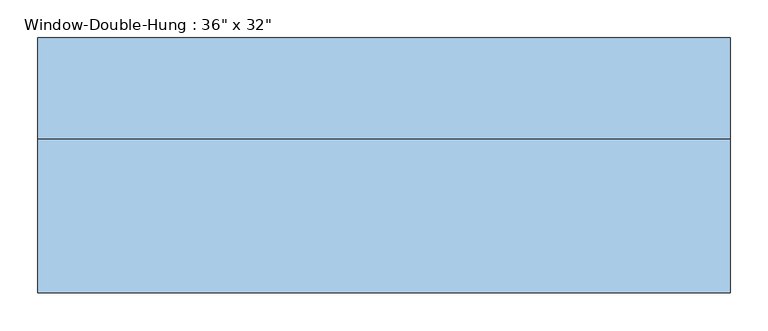
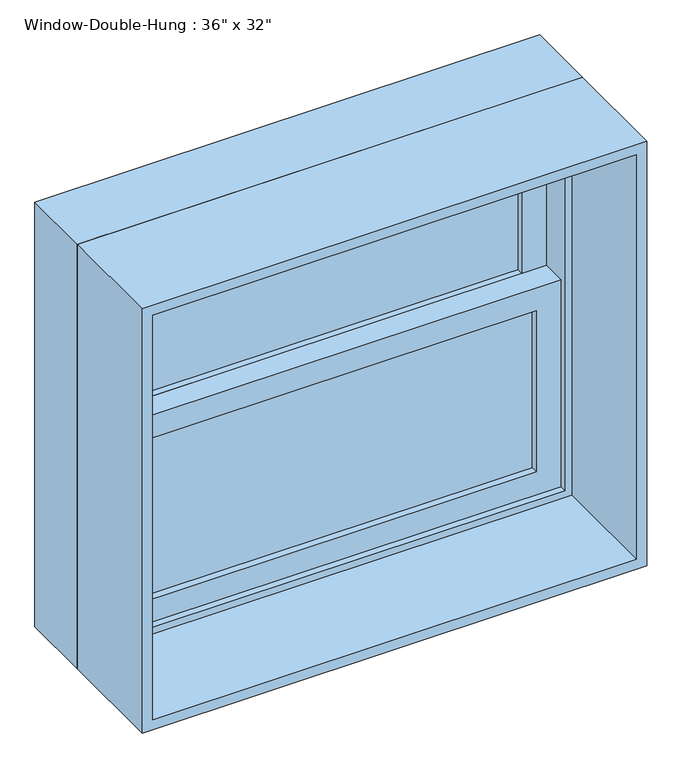
"""IFC4 building model written with IfcOpenShell, lengths in millimetres: window geometry."""

from ifc_helpers import new_model, si_unit, frame, origin, place, context, project, spatial, polyline, outline, extrude, source, transform, mapped, element, save


def window_21393ef8(model_context):
    return source(origin(), model_context, "Body", "SweptSolid", [
        extrude(outline(polyline([(381.0, 88.9), (381.0, 82.55), (-381.0, 82.55), (-381.0, 88.9), (381.0, 88.9)])), frame((0.0, 0.0, 990.6), z_axis=(0.0, 0.0, 1.0), x_axis=(1.0, 0.0, 0.0)), (0.0, 0.0, 1.0), 307.975),
        extrude(outline(polyline([(-381.0, 76.2), (381.0, 76.2), (381.0, 69.85), (-381.0, 69.85), (-381.0, 76.2)])), frame((0.0, 0.0, 990.6), z_axis=(0.0, 0.0, 1.0), x_axis=(1.0, 0.0, 0.0)), (0.0, 0.0, 1.0), 307.975),
        extrude(outline(polyline([(381.0, 133.35), (381.0, 127.0), (-381.0, 127.0), (-381.0, 133.35), (381.0, 133.35)])), frame((0.0, 0.0, 1343.025), z_axis=(0.0, 0.0, 1.0), x_axis=(1.0, 0.0, 0.0)), (0.0, 0.0, 1.0), 307.975),
        extrude(outline(polyline([(-381.0, 120.65), (381.0, 120.65), (381.0, 114.3), (-381.0, 114.3), (-381.0, 120.65)])), frame((0.0, 0.0, 1343.025), z_axis=(0.0, 0.0, 1.0), x_axis=(1.0, 0.0, 0.0)), (0.0, 0.0, 1.0), 307.975),
        extrude(outline(polyline([(1343.025, -425.45), (946.15, -425.45), (946.15, 425.45), (1343.025, 425.45), (1343.025, -425.45)]), holes=[polyline([(1298.575, 381.0), (990.6, 381.0), (990.6, -381.0), (1298.575, -381.0), (1298.575, 381.0)])]), frame((0.0, 57.15, 0.0), z_axis=(0.0, 1.0, 0.0), x_axis=(0.0, 0.0, 1.0)), (0.0, 0.0, 1.0), 44.45),
        extrude(outline(polyline([(1695.45, -425.45), (1298.575, -425.45), (1298.575, 425.45), (1695.45, 425.45), (1695.45, -425.45)]), holes=[polyline([(1651.0, 381.0), (1343.025, 381.0), (1343.025, -381.0), (1651.0, -381.0), (1651.0, 381.0)])]), frame((0.0, 101.6, 0.0), z_axis=(0.0, 1.0, 0.0), x_axis=(0.0, 0.0, 1.0)), (0.0, 0.0, 1.0), 44.45),
        extrude(outline(polyline([(1727.2, -457.2), (914.4, -457.2), (914.4, 457.2), (1727.2, 457.2), (1727.2, -457.2)]), holes=[polyline([(1695.45, 425.45), (946.15, 425.45), (946.15, -425.45), (1695.45, -425.45), (1695.45, 425.45)])]), frame((0.0, 44.45, 0.0), z_axis=(0.0, 1.0, 0.0), x_axis=(0.0, 0.0, 1.0)), (0.0, 0.0, 1.0), 133.35),
        extrude(outline(polyline([(1727.2, 457.2), (1727.2, -457.2), (914.4, -457.2), (914.4, 457.2), (1727.2, 457.2)]), holes=[polyline([(1708.15, 438.15), (933.45, 438.15), (933.45, -438.15), (1708.15, -438.15), (1708.15, 438.15)])]), frame((0.0, -158.75, 0.0), z_axis=(0.0, 1.0, 0.0), x_axis=(0.0, 0.0, 1.0)), (0.0, 0.0, 1.0), 203.2),
    ])


if __name__ == "__main__":
    model = new_model("IFC4")
    model_context = context("Model", 3, world=origin())
    ifc_project = project(units=[si_unit("LENGTHUNIT", "METRE", prefix="MILLI")], contexts=[model_context])
    site = spatial("IfcSite", under=ifc_project)
    building = spatial("IfcBuilding", under=site)
    placement = place(None, origin())
    window_shape = window_21393ef8(model_context)
    element("IfcWindow", 1, ObjectType="Window-Double-Hung : 36\" x 32\"", at=placement, inside=building, context=model_context, shape_type="MappedRepresentation", body=[
        mapped(window_shape, transform((0.0, 0.0, 0.0), x_axis=(1.0, 0.0, 0.0), y_axis=(0.0, 1.0, 0.0), z_axis=(0.0, 0.0, 1.0))),
    ])
    save(model, "model.ifc")

# Revit data of these elements
# Type "Window-Double-Hung : 36\" x 32\""
#   Type Mark = "19"
#   Fire Rating = "0.5h"
#   Construction Type Id = "DG-DR"
#   Assembly Code = "B2020100"
#   Analytic Construction = "Double glazing - domestic"
#   Wall Thickness [instance default] = 0' - 6"
#   Window Inset [instance default] = 0' - 0"
#   Visual Light Transmittance = 0.81
#   Thermal Resistance (R) = 1.8146 (h·ft²·°F)/BTU
#   Solar Heat Gain Coefficient = 0.76
#   Muntin Width = 2' - 6"
#   Muntin Height = 1' - 0 1/8"
#   Interior Wall Closure [instance default] = 0' - 1 1/2"
#   Rough Width = 3' - 0 1/2"
#   Rough Height = 2' - 8 1/2"
#   Frame Extension [instance default] = 0' - 1 1/4"
#   Exterior Wall Closure [instance default] = 0' - 0 1/2"
#   Extension Jamb [instance default] = 0' - 1 1/2"
#   Heat Transfer Coefficient (U) = 0.5511 BTU/(h·ft²·°F)
#   Height = 2' - 8"
#   Width = 3' - 0"
#   Top Muntin Visibility = yes
#   Indicator Visibility [instance default] = yes
#   Extension Jamb Visibility [instance default] = yes
#   Interior Trim Visibility [instance default] = yes
#   Exterior Trim Visibility [instance default] = yes
#   Define Thermal Properties by = 1
#   Bottom Muntin Visibility = yes
#   Muntin Pattern = Muntin Pattern_2x2 : Muntin Pattern_2x2
#   Interior Trim Material = Maple - Semigloss(Rotated)
#   Interior Trim = Trim-Window-Interior-Flat : Picture Frame
#   Exterior Trim Material = Clad - White
#   Exterior Trim = Trim-Window-Exterior-Flat : with Sill
#   Glass Panel Material = Glass, Clear Glazing
#   Exterior Frame Material = Clad - White
#   Interior Frame Material = Maple - Semigloss(Rotated)
#   Wall Closure = (empty or 0)
# Element 1 (IfcWindow, "Window-Double-Hung : 36\" x 32\"")
#   Wall Thickness = 1' - 0 1/2"
#   Extension Jamb = 0' - 8"
#   Materials on its faces: "Maple - Semigloss(Rotated)", "Glass, Clear Glazing", "Clad - White"
# Materials
#   "Maple - Semigloss(Rotated)": class "Wood", colour RGB 196 161 118, transparency 0, Description = "Acer Saccharum", Cost = 0
#   "Clad - White": class "Wood", colour RGB 245 245 243, transparency 0, Cost = 0
#   "Glass, Clear Glazing": class "Glass", colour RGB 245 245 243, transparency 1, Description = "Clear glazing", Cost = 0
